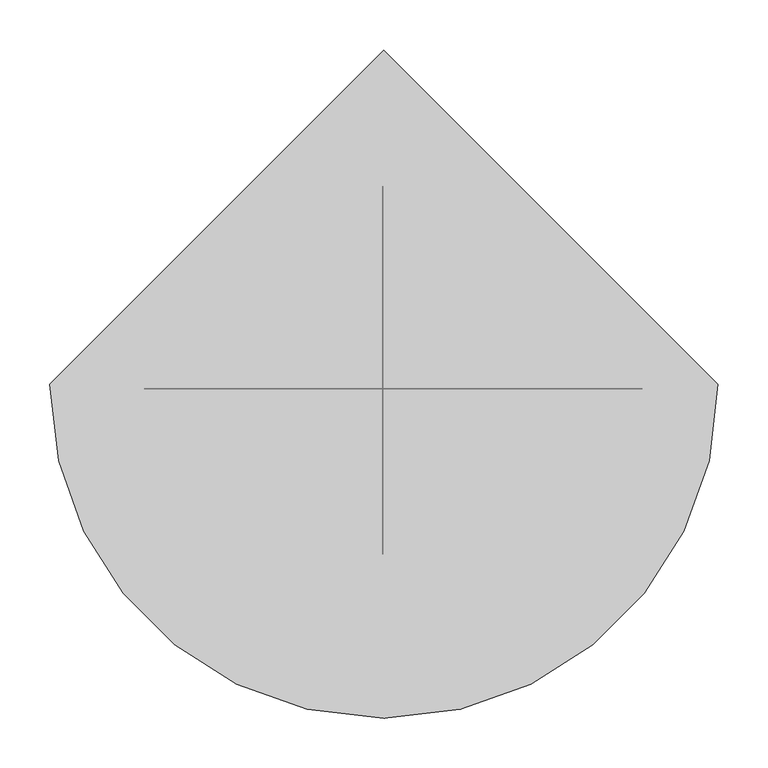
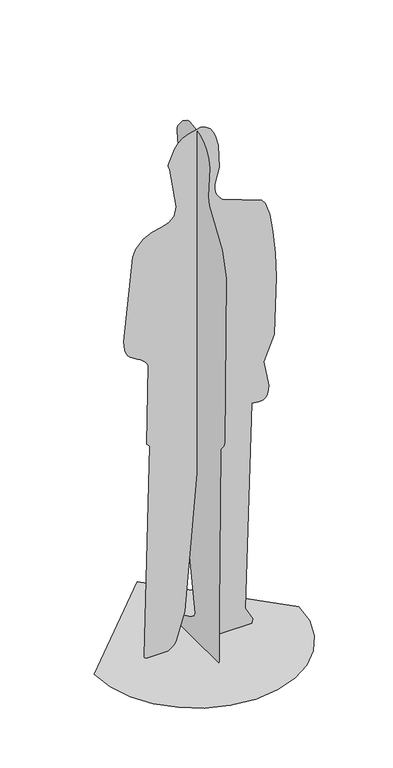
"""IFC4 building model written with IfcOpenShell, lengths in millimetres: proxy geometry, dwayne 23733 : dwayne 23733."""

from ifc_helpers import new_model, si_unit, origin, place, context, project, spatial, triangles, source, transform, mapped, element, save


def entourage_8da15c99(model_context):
    return source(origin(), model_context, "Body", "Tessellation", [
        triangles([(-180.7520848, -4.45e-05, 5.61e-05), (-184.2428783, -8.8e-06, 2.7953159), (-186.1722845, 1.66e-05, 5.8375037), (-186.8317464, 3.35e-05, 9.1275741), (-168.2847317, 8.5e-06, 733.0655743), (-173.8813923, 8.5e-06, 735.2245268), (-177.6699692, 8.1e-06, 740.933626), (-174.1986513, -8.1e-06, 1013.6688681), (-179.5913999, -8.8e-06, 1024.1657564), (-188.0396306, -9.6e-06, 1032.776568), (-198.5268356, -9.9e-06, 1040.1131842), (-210.0364347, -1.03e-05, 1046.7870501), (-221.5521744, -1.07e-05, 1053.4099016), (-232.0573471, -1.1e-05, 1060.5935474), (-240.5355178, -1.14e-05, 1068.9495054), (-245.9520113, -1.21e-05, 1078.9886456), (-249.7388442, -1.29e-05, 1091.9828379), (-252.1553936, -1.4e-05, 1106.9305447), (-253.4609098, -1.47e-05, 1122.8302282), (-224.2189811, -3.16e-05, 1405.0555161), (-213.7950534, -3.31e-05, 1430.2028183), (-189.1320784, -3.46e-05, 1456.0851048), (-160.6250248, -3.53e-05, 1468.8744404), (-131.9230613, -3.57e-05, 1475.6387077), (-106.6753564, -3.64e-05, 1483.4444813), (-88.5310787, -3.71e-05, 1499.3602249), (-81.1393152, -3.9e-05, 1530.4525131), (-102.9420995, -4.71e-05, 1666.4706642), (-107.9473082, -4.78e-05, 1679.2661041), (-108.147514, -4.82e-05, 1680.5750359), (-107.9848786, -4.82e-05, 1682.7597862), (-107.5268942, -4.82e-05, 1685.5199375), (-106.8410076, -4.86e-05, 1688.5562347), (-86.6409597, -5.11e-05, 1733.0913071), (-74.2774747, -5.19e-05, 1747.7193386), (-59.5121968, -5.26e-05, 1759.6604702), (-42.3631437, -5.33e-05, 1768.778809), (-0.985526, -5.37e-05, 1778.0000484), (15.8808848, -5.33e-05, 1772.5538692), (29.1619713, -5.26e-05, 1761.5650051), (39.2640596, -5.19e-05, 1747.0972836), (46.5934905, -5.08e-05, 1731.2151134), (56.0091948, -4.89e-05, 1695.7216404), (59.1639804, -4.41e-05, 1618.2096565), (44.4858611, -4.12e-05, 1564.728764), (44.3096955, -4.05e-05, 1551.1871487), (46.5533085, -3.94e-05, 1537.928801), (51.2886617, -3.86e-05, 1525.4368309), (58.5876893, -3.83e-05, 1514.1934765), (68.5223573, -3.75e-05, 1504.6817024), (198.4031332, -3.46e-05, 1454.5817081), (210.7096676, -3.38e-05, 1440.8303673), (224.9007164, -3.13e-05, 1397.8456364), (235.5370584, -2.72e-05, 1333.6076969), (242.7581838, -2.28e-05, 1256.1539944), (246.7033826, -1.77e-05, 1173.5217562), (240.2782843, -5.9e-06, 974.9295902), (206.0815162, -1.1e-06, 891.6227566), (221.1963095, 4e-06, 805.6638319), (220.4651949, 5.1e-06, 788.6204681), (214.9949983, 6.3e-06, 771.8049974), (210.3553288, 6.6e-06, 765.7305136), (204.1669347, 6.6e-06, 762.0923635), (196.896103, 7e-06, 760.3986443), (189.0091026, 7e-06, 760.1578159), (180.9722385, 7e-06, 760.8779028), (173.2516706, 6.6e-06, 762.0673651), (166.3136674, 6.6e-06, 763.2343723), (144.8011997, 4.49e-05, 59.4753214), (168.6276432, 4.74e-05, 15.3365923), (166.1986854, -4.45e-05, 5.61e-05), (66.1332453, -4.45e-05, 5.61e-05), (49.8425291, -1.03e-05, 3.9765614), (39.0246438, 1.36e-05, 14.0353079), (32.5983191, 2.91e-05, 28.3297275), (-2.744106, 9.2e-06, 720.0463108), (-54.0725352, 1.03e-05, 117.9433913), (-81.3720589, -2.13e-05, 28.0047586), (-85.5237496, -2.69e-05, 19.9172799), (-91.2434313, -3.27e-05, 12.5691251), (-99.2452049, -3.86e-05, 5.9378921), (-110.2432618, -4.45e-05, 5.61e-05), (-13.8237486, -127.6719491, 9.9621213), (-13.8238053, -127.261836, 182.0843436), (-13.8237894, -135.2636459, 744.8700136), (-13.8237894, -136.4150655, 748.3464729), (-13.8237894, -139.3955521, 752.5740492), (-13.8237894, -143.4944844, 757.5063063), (-13.8237894, -148.0011678, 763.0967354), (-13.8237894, -152.2050719, 769.2988277), (-13.8237872, -155.3954567, 776.0660746), (-13.8237872, -156.8617189, 783.3521124), (-13.8237701, -165.9465932, 1358.6144554), (-13.8237679, -143.2744033, 1442.0936623), (-13.8237656, -71.1145909, 1552.8595757), (-13.8237656, -64.3402088, 1580.52155), (-13.8237622, -73.5344423, 1684.7962898), (-13.823761, -67.2131621, 1712.2171452), (-13.823761, -55.2412548, 1734.9080566), (-13.823761, -37.926044, 1752.7547871), (-13.823761, -15.5748862, 1765.6435352), (-13.823761, 11.5049153, 1773.4603546), (-13.823761, 43.0060141, 1776.0911533), (-13.823761, 55.0860544, 1772.9175098), (-13.8237622, 79.7039013, 1756.3228832), (-13.8237633, 107.489678, 1722.3487942), (-13.8237633, 111.5712331, 1713.0111374), (-13.8237633, 112.222992, 1702.3029247), (-13.8237667, 99.0832871, 1611.9293713), (-13.8237667, 100.6007817, 1597.8216568), (-13.8237679, 96.7552315, 1579.0665516), (-13.8237701, 31.1784748, 1488.4601635), (-13.8237815, 125.7984987, 1146.7478817), (-13.8237815, 134.1994394, 1137.675761), (-13.8237826, 184.2800127, 1119.3932287), (-13.8237826, 194.4650741, 1111.9401226), (-13.8237826, 201.1344345, 1100.3807991), (-13.8237849, 203.5509657, 1084.206423), (-13.8237849, 200.9675115, 1068.9646208), (-13.8237849, 194.2821819, 1055.8713066), (-13.8237849, 184.3929236, 1046.1421766), (-13.8237849, 172.1979195, 1040.9932903), (-13.8237849, 158.5950979, 1041.6405619), (-13.8237849, 144.4825418, 1049.2996874), (-13.8237917, 123.0430165, 785.7652645), (-13.8237928, 116.9063816, 707.2433859), (-13.8238008, 10.2023739, 90.6853713), (-13.8238019, 17.9839052, 76.1482317), (-13.8238031, 35.4714609, 63.8067794), (-13.8238121, 104.5965861, 31.8661645), (-13.8238133, 119.3345128, 20.2173774), (-13.8238155, 122.9915752, 6.7192125), (-13.8238121, 122.0607817, 4.3675023), (-13.8237974, 120.3452433, 2.3141491), (-13.8237803, 119.1854304, 1.4285661), (-13.8237542, 117.8200159, 0.6534775), (-13.8237179, 116.2459023, 5.61e-05), (-13.8237156, -124.5016756, 0.0), (-348.4736423, 4.7230064, 0.0001684), (-339.5989297, -72.1961928, 0.0001684), (-314.3239463, -142.8341776, 5.61e-05), (-274.6723876, -205.1670917, 5.61e-05), (-222.6682945, -257.1712393, 5.61e-05), (-160.3353441, -296.8226708, 5.61e-05), (-89.6973684, -322.0977087, 5.61e-05), (-12.7781717, -330.9724577, 5.61e-05), (64.1410249, -322.097745, 5.61e-05), (134.7790189, -296.8227253, 5.61e-05), (197.1119329, -257.171203, 5.61e-05), (249.1161351, -205.167128, 5.61e-05), (288.7675302, -142.8341413, 5.61e-05), (314.0425681, -72.1961383, 0.0001684), (322.9173171, 4.7230359, 0.0001684), (-12.7782308, 340.4184654, 0.0001684)], [[70, 71, 72], [69, 70, 72], [69, 72, 73], [69, 73, 74], [69, 74, 75], [69, 75, 76], [68, 69, 76], [82, 1, 2], [82, 2, 3], [82, 3, 4], [81, 82, 4], [80, 81, 4], [79, 80, 4], [78, 79, 4], [77, 78, 4], [77, 4, 5], [76, 77, 5], [5, 6, 7], [76, 5, 7], [76, 7, 8], [68, 76, 8], [67, 68, 8], [66, 67, 8], [65, 66, 8], [64, 65, 8], [63, 64, 8], [62, 63, 8], [61, 62, 8], [60, 61, 8], [59, 60, 8], [58, 59, 8], [57, 58, 8], [56, 57, 8], [56, 8, 9], [55, 56, 9], [55, 9, 10], [54, 55, 10], [54, 10, 11], [53, 54, 11], [53, 11, 12], [52, 53, 12], [51, 52, 12], [50, 51, 12], [50, 12, 13], [50, 13, 14], [50, 14, 15], [50, 15, 16], [50, 16, 17], [50, 17, 18], [50, 18, 19], [50, 19, 20], [50, 20, 21], [50, 21, 22], [50, 22, 23], [50, 23, 24], [50, 24, 25], [50, 25, 26], [49, 50, 26], [48, 49, 26], [48, 26, 27], [47, 48, 27], [46, 47, 27], [45, 46, 27], [44, 45, 27], [44, 27, 28], [43, 44, 28], [42, 43, 28], [42, 28, 29], [42, 29, 30], [42, 30, 31], [42, 31, 32], [42, 32, 33], [42, 33, 34], [42, 34, 35], [42, 35, 36], [42, 36, 37], [41, 42, 37], [40, 41, 37], [40, 37, 38], [40, 38, 39], [137, 138, 83], [137, 83, 84], [136, 137, 84], [135, 136, 84], [130, 131, 132], [130, 132, 133], [130, 133, 134], [130, 134, 135], [122, 123, 124], [121, 122, 124], [120, 121, 124], [119, 120, 124], [118, 119, 124], [117, 118, 124], [116, 117, 124], [115, 116, 124], [114, 115, 124], [113, 114, 124], [106, 107, 108], [105, 106, 108], [104, 105, 108], [103, 104, 108], [102, 103, 108], [101, 102, 108], [100, 101, 108], [99, 100, 108], [98, 99, 108], [97, 98, 108], [97, 108, 109], [97, 109, 110], [97, 110, 111], [96, 97, 111], [95, 96, 111], [95, 111, 112], [94, 95, 112], [93, 94, 112], [93, 112, 113], [92, 93, 113], [92, 113, 124], [92, 124, 125], [91, 92, 125], [90, 91, 125], [89, 90, 125], [88, 89, 125], [87, 88, 125], [86, 87, 125], [86, 125, 126], [85, 86, 126], [85, 126, 127], [84, 85, 127], [84, 127, 128], [135, 84, 128], [135, 128, 129], [130, 135, 129], [153, 154, 139], [152, 153, 139], [152, 139, 140], [151, 152, 140], [151, 140, 141], [151, 141, 142], [150, 151, 142], [149, 150, 142], [149, 142, 143], [149, 143, 144], [149, 144, 145], [149, 145, 146], [149, 146, 147], [149, 147, 148]], closed=False),
    ])


if __name__ == "__main__":
    model = new_model("IFC4")
    model_context = context("Model", 3, world=origin())
    ifc_project = project(units=[si_unit("LENGTHUNIT", "METRE", prefix="MILLI")], contexts=[model_context])
    site = spatial("IfcSite", under=ifc_project)
    building = spatial("IfcBuilding", under=site)
    placement = place(None, origin())
    entourage_shape = entourage_8da15c99(model_context)
    element("IfcBuildingElementProxy", 1, Name="dwayne 23733 : dwayne 23733", ObjectType="dwayne 23733 : dwayne 23733", at=placement, inside=building, context=model_context, shape_type="MappedRepresentation", body=[
        mapped(entourage_shape, transform((0.0, 0.0, 0.0), x_axis=(1.0, 0.0, 0.0), y_axis=(0.0, 1.0, 0.0), z_axis=(0.0, 0.0, 1.0))),
    ])
    save(model, "model.ifc")

# Revit data of these elements
# Type "dwayne 23733 : dwayne 23733"
#   built-in parameter 1005195 = "RPC-8-G1AE-S4G0-CKUK-A"
#   Height = 0
